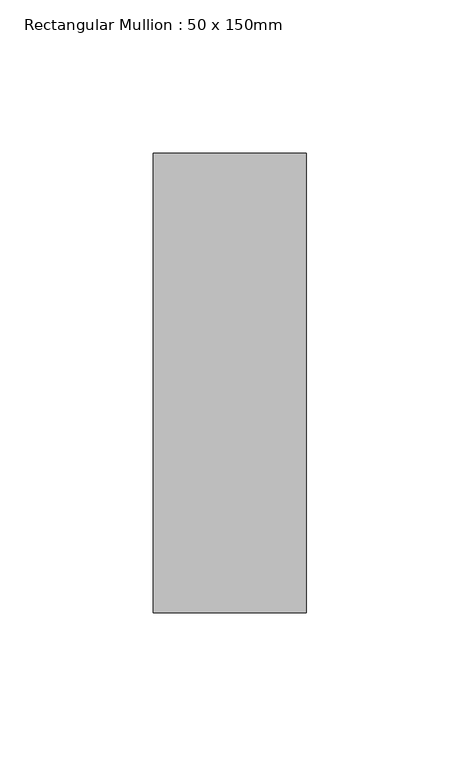
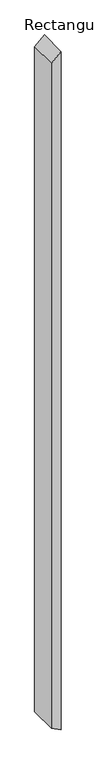
"""IFC4 building model written with IfcOpenShell, lengths in millimetres: member geometry, Rectangular Mullion : 50 x 150mm."""

from ifc_helpers import new_model, si_unit, frame, origin, place, context, project, spatial, polyline, outline, extrude, source, transform, mapped, element, save


def rectangular_mullion_50_x_150mm_139992b9(model_context):
    return source(origin(), model_context, "Body", "SweptSolid", [
        extrude(outline(polyline([(0.0, 0.0), (-47.0734921, -50.0), (-3684.0028111, -50.0), (-3710.9535778, 0.0), (0.0, 0.0)])), frame((0.0, -75.0, 0.0), z_axis=(0.0, 1.0, 0.0), x_axis=(0.0, 0.0, 1.0)), (0.0, 0.0, 1.0), 150.0),
    ])


if __name__ == "__main__":
    model = new_model("IFC4")
    model_context = context("Model", 3, world=origin())
    ifc_project = project(units=[si_unit("LENGTHUNIT", "METRE", prefix="MILLI")], contexts=[model_context])
    site = spatial("IfcSite", under=ifc_project)
    building = spatial("IfcBuilding", under=site)
    placement = place(None, origin())
    rectangular_mullion_50_x_150mm_shape = rectangular_mullion_50_x_150mm_139992b9(model_context)
    element("IfcMember", 1, ObjectType="Rectangular Mullion : 50 x 150mm", at=placement, inside=building, context=model_context, shape_type="MappedRepresentation", body=[
        mapped(rectangular_mullion_50_x_150mm_shape, transform((0.0, 0.0, 0.0), x_axis=(1.0, 0.0, 0.0), y_axis=(0.0, 1.0, 0.0), z_axis=(0.0, 0.0, 1.0))),
    ])
    save(model, "model.ifc")

# Revit data of these elements
# Type "Rectangular Mullion : 50 x 150mm"
#   built-in parameter 1007304 = 0.492126 (stored number, unit not read)
#   built-in parameter 1007301 = 0.082021 (stored number, unit not read)
#   built-in parameter 1007300 = 0.082021 (stored number, unit not read)
# Element 1 (IfcMember, "Rectangular Mullion : 50 x 150mm")
#   Materials on its faces: "Metal - Aluminium"
# Materials
#   "Metal - Aluminium": class "Metal", colour RGB 247 247 247, transparency 0
